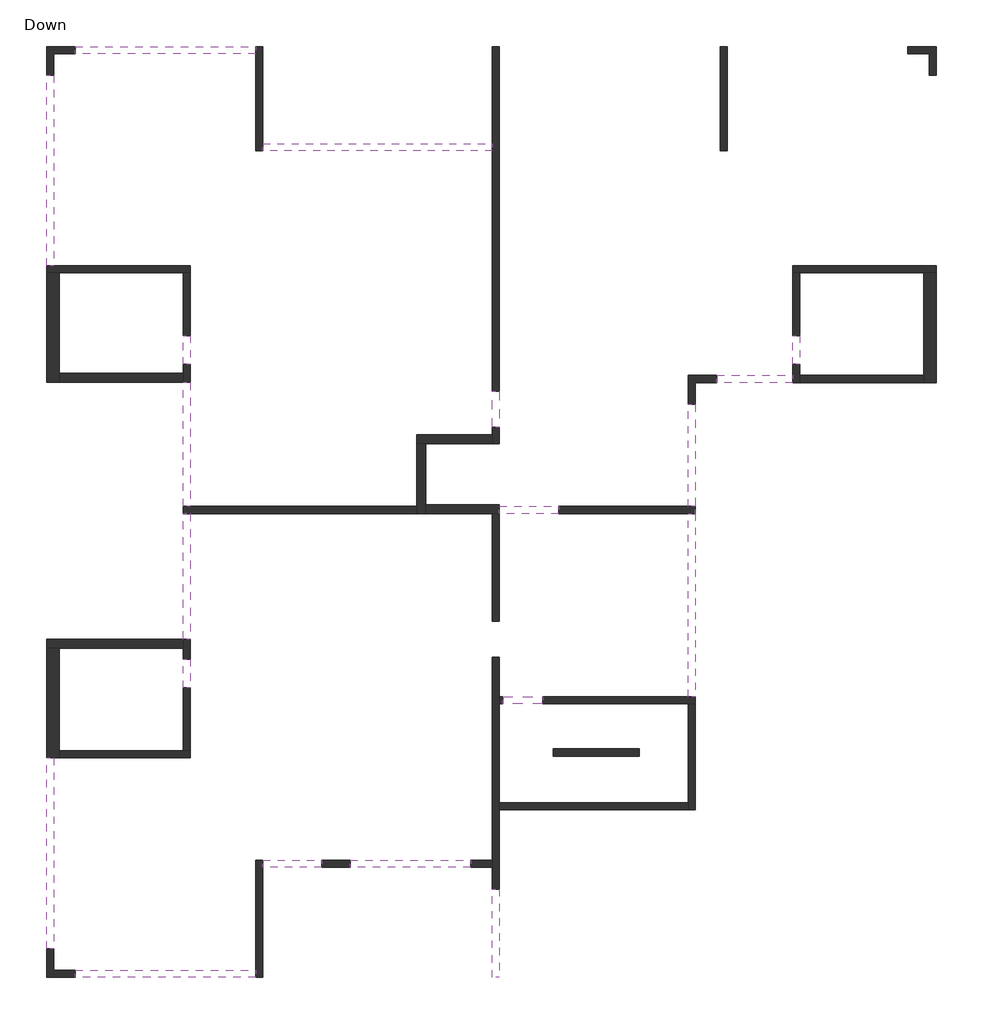
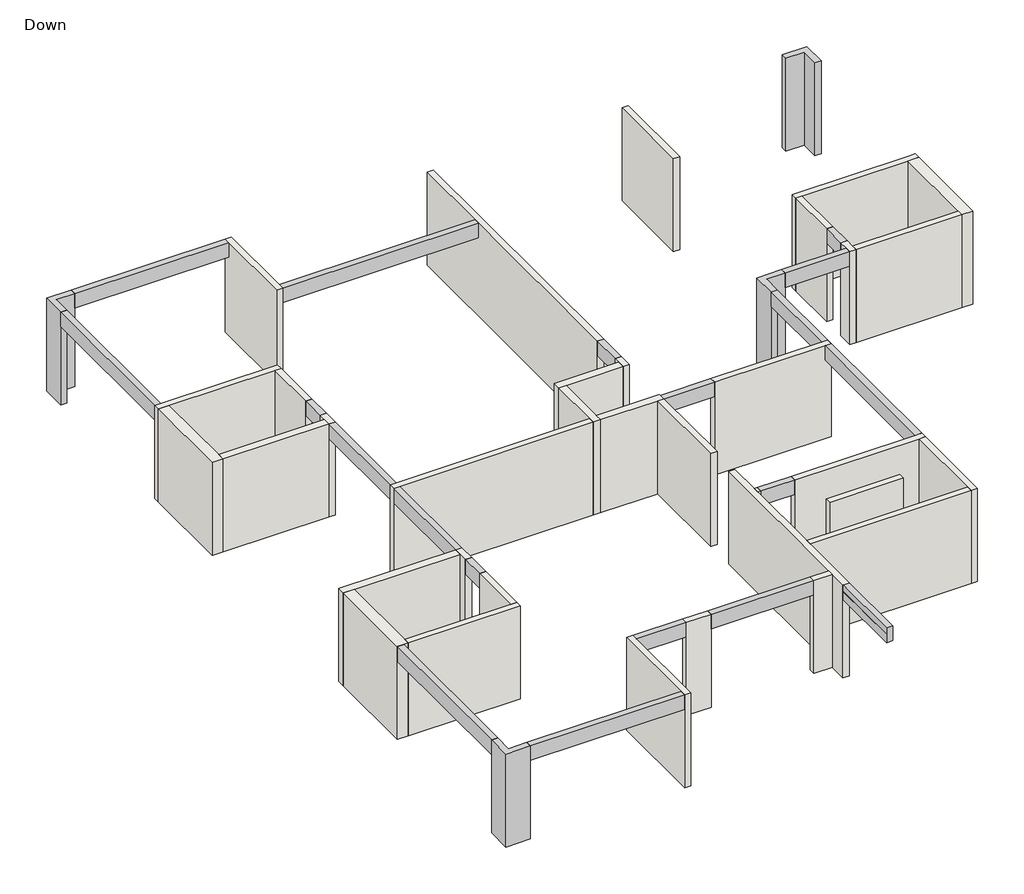
# One storey: 34 walls, 19 beams, 4 columns.
# Revit data of these elements (continued)
# Element 30 (IfcWall, "20") (continued)
#   Base Constraint = Down
#   Top Constraint = Typical Floor
#   Materials on its faces: "Concrete"
# Element 31 (IfcWall, "20")
#   Comments = ""
#   Mark = "W8"
#   SOFiSTiK_EdgeZones = "W8"
#   SOFiSTiK_AMG_Comments = ""
#   Top Offset = 0 cm
#   Base Offset = 0 cm
#   wall height = 320 cm
#   SOFiSTiK_AMG_Scheduled = yes
#   SOFiSTiK_AMG_Adjusted = yes
#   Phase Created = New Construction
#   Base Constraint = Down
#   Top Constraint = Typical Floor
#   Materials on its faces: "Concrete"
# Element 32 (IfcWall, "20")
#   Comments = ""
#   Mark = "W9"
#   SOFiSTiK_EdgeZones = "W9"
#   SOFiSTiK_AMG_Comments = ""
#   Top Offset = 0 cm
#   Base Offset = 0 cm
#   wall height = 320 cm
#   SOFiSTiK_AMG_Scheduled = yes
#   SOFiSTiK_AMG_Adjusted = yes
#   Phase Created = New Construction
#   Base Constraint = Down
#   Top Constraint = Typical Floor
#   Materials on its faces: "Concrete"
# Element 33 (IfcWall, "20")
#   Comments = ""
#   Mark = "W10"
#   SOFiSTiK_EdgeZones = "W10"
#   SOFiSTiK_AMG_Comments = ""
#   Top Offset = 0 cm
#   Base Offset = 0 cm
#   wall height = 320 cm
#   SOFiSTiK_AMG_Scheduled = yes
#   SOFiSTiK_AMG_Adjusted = yes
#   Phase Created = New Construction
#   Base Constraint = Down
#   Top Constraint = Typical Floor
#   Materials on its faces: "Concrete"
# Element 34 (IfcWall, "20")
#   Comments = ""
#   Mark = "W11"
#   SOFiSTiK_EdgeZones = "W11"
#   SOFiSTiK_AMG_Comments = ""
#   Top Offset = 0 cm
#   Base Offset = 0 cm
#   wall height = 320 cm
#   SOFiSTiK_AMG_Scheduled = yes
#   SOFiSTiK_AMG_Adjusted = yes
#   Phase Created = New Construction
#   Base Constraint = Down
#   Top Constraint = Typical Floor
#   Materials on its faces: "Concrete"
# Element 35 (IfcWall, "20")
#   Comments = ""
#   Mark = "W12"
#   SOFiSTiK_EdgeZones = "W12"
#   SOFiSTiK_AMG_Comments = ""
#   Top Offset = 0 cm
#   Base Offset = 0 cm
#   wall height = 320 cm
#   SOFiSTiK_AMG_Scheduled = yes
#   SOFiSTiK_AMG_Adjusted = yes
#   Phase Created = New Construction
#   Base Constraint = Down
#   Top Constraint = Typical Floor
#   Materials on its faces: "Concrete"
# Element 36 (IfcWall, "20")
#   Comments = ""
#   Mark = "W13"
#   SOFiSTiK_EdgeZones = "W13"
#   SOFiSTiK_AMG_Comments = ""
#   Top Offset = 0 cm
#   Base Offset = 0 cm
#   wall height = 320 cm
#   SOFiSTiK_AMG_Scheduled = yes
#   SOFiSTiK_AMG_Adjusted = yes
#   Phase Created = New Construction
#   Base Constraint = Down
#   Top Constraint = Typical Floor
#   Materials on its faces: "Concrete"
# Element 37 (IfcWall, "20")
#   Comments = ""
#   Mark = "W14"
#   SOFiSTiK_EdgeZones = "W14"
#   SOFiSTiK_AMG_Comments = ""
#   Top Offset = 0 cm
#   Base Offset = 0 cm
#   wall height = 320 cm
#   SOFiSTiK_AMG_Scheduled = yes
#   SOFiSTiK_AMG_Adjusted = yes
#   Phase Created = New Construction
#   Base Constraint = Down
#   Top Constraint = Typical Floor
#   Materials on its faces: "Concrete"
# Element 38 (IfcWall, "20")
#   Comments = ""
#   Mark = "W15"
#   SOFiSTiK_EdgeZones = "W15"
#   SOFiSTiK_AMG_Comments = ""
#   Top Offset = 0 cm
#   Base Offset = 0 cm
#   wall height = 320 cm
#   SOFiSTiK_AMG_Scheduled = yes
#   SOFiSTiK_AMG_Adjusted = yes
#   Phase Created = New Construction
#   Base Constraint = Down
#   Top Constraint = Typical Floor
#   Materials on its faces: "Concrete"
# Element 39 (IfcWall, "20")
#   Comments = ""
#   Mark = "W16"
#   SOFiSTiK_EdgeZones = "W16"
#   SOFiSTiK_AMG_Comments = ""
#   Top Offset = 0 cm
#   Base Offset = 0 cm
#   wall height = 320 cm
#   SOFiSTiK_AMG_Scheduled = yes
#   SOFiSTiK_AMG_Adjusted = yes
#   Phase Created = New Construction
#   Base Constraint = Down
#   Top Constraint = Typical Floor
#   Materials on its faces: "Concrete"
# Element 40 (IfcWall, "20")
#   Comments = ""
#   Mark = "W17"
#   SOFiSTiK_EdgeZones = "W17"
#   SOFiSTiK_AMG_Comments = ""
#   Top Offset = 0 cm
#   Base Offset = 0 cm
#   wall height = 320 cm
#   SOFiSTiK_AMG_Scheduled = yes
#   SOFiSTiK_AMG_Adjusted = yes
#   Phase Created = New Construction
#   Base Constraint = Down
#   Top Constraint = Typical Floor
#   Materials on its faces: "Concrete"
# Element 41 (IfcWall, "20")
#   Comments = ""
#   Mark = "W18"
#   SOFiSTiK_EdgeZones = "W18"
#   SOFiSTiK_AMG_Comments = ""
#   Top Offset = 0 cm
#   Base Offset = 0 cm
#   wall height = 320 cm
#   SOFiSTiK_AMG_Scheduled = yes
#   SOFiSTiK_AMG_Adjusted = yes
#   Phase Created = New Construction
#   Base Constraint = Down
#   Top Constraint = Typical Floor
#   Materials on its faces: "Concrete"
# Element 42 (IfcWall, "20")
#   Comments = ""
#   Mark = "W19"
#   SOFiSTiK_EdgeZones = "W19"
#   SOFiSTiK_AMG_Comments = "Too Short /"
#   Top Offset = 0 cm
#   Base Offset = 0 cm
#   wall height = 320 cm
#   SOFiSTiK_AMG_Scheduled = yes
#   SOFiSTiK_AMG_Adjusted = yes
#   Phase Created = New Construction
#   Base Constraint = Down
#   Top Constraint = Typical Floor
#   Materials on its faces: "Concrete"
# Element 43 (IfcWall, "20")
#   Comments = ""
#   Mark = "W20"
#   SOFiSTiK_EdgeZones = "W20"
#   SOFiSTiK_AMG_Comments = ""
#   Top Offset = 0 cm
#   Base Offset = 0 cm
#   wall height = 320 cm
#   SOFiSTiK_AMG_Scheduled = yes
#   SOFiSTiK_AMG_Adjusted = yes
#   Phase Created = New Construction
#   Base Constraint = Down
#   Top Constraint = Typical Floor
#   Materials on its faces: "Concrete"
# Element 44 (IfcWall, "20")
#   Comments = ""
#   Mark = "W21"
#   SOFiSTiK_EdgeZones = "W21"
#   SOFiSTiK_AMG_Comments = ""
#   Top Offset = 0 cm
#   Base Offset = 0 cm
#   wall height = 320 cm
#   SOFiSTiK_AMG_Scheduled = yes
#   SOFiSTiK_AMG_Adjusted = yes
#   Phase Created = New Construction
#   Base Constraint = Down
#   Top Constraint = Typical Floor
#   Materials on its faces: "Concrete"
# Element 45 (IfcWall, "20")
#   Comments = ""
#   Mark = "W22"
#   SOFiSTiK_EdgeZones = "W22"
#   SOFiSTiK_AMG_Comments = ""
#   Top Offset = 0 cm
#   Base Offset = 0 cm
#   wall height = 320 cm
#   SOFiSTiK_AMG_Scheduled = yes
#   SOFiSTiK_AMG_Adjusted = yes
#   Phase Created = New Construction
#   Base Constraint = Down
#   Top Constraint = Typical Floor
#   Materials on its faces: "Concrete"
# Element 46 (IfcWall, "20")
#   Comments = ""
#   Mark = "W23"
#   SOFiSTiK_EdgeZones = "W23"
#   SOFiSTiK_AMG_Comments = ""
#   Top Offset = 0 cm
#   Base Offset = 0 cm
#   wall height = 320 cm
#   SOFiSTiK_AMG_Scheduled = yes
#   SOFiSTiK_AMG_Adjusted = yes
#   Phase Created = New Construction
#   Base Constraint = Down
#   Top Constraint = Typical Floor
#   Materials on its faces: "Concrete"
# Element 47 (IfcWall, "20")
#   Comments = ""
#   Mark = "W24"
#   SOFiSTiK_EdgeZones = "W24"
#   SOFiSTiK_AMG_Comments = ""
#   Top Offset = 0 cm
#   Base Offset = 0 cm
#   wall height = 320 cm
#   SOFiSTiK_AMG_Scheduled = yes
#   SOFiSTiK_AMG_Adjusted = yes
#   Phase Created = New Construction
#   Base Constraint = Down
#   Top Constraint = Typical Floor
#   Materials on its faces: "Concrete"
# Element 48 (IfcWall, "20")
#   Comments = ""
#   Mark = "W25"
#   SOFiSTiK_EdgeZones = "W25"
#   SOFiSTiK_AMG_Comments = ""
#   Top Offset = 0 cm
#   Base Offset = 0 cm
#   wall height = 320 cm
#   SOFiSTiK_AMG_Scheduled = yes
#   SOFiSTiK_AMG_Adjusted = yes
#   Phase Created = New Construction
#   Base Constraint = Down
#   Top Constraint = Typical Floor
#   Materials on its faces: "Concrete"
# Element 49 (IfcWall, "20")
#   Comments = ""
#   Mark = "W26"
#   SOFiSTiK_EdgeZones = "W26"
#   SOFiSTiK_AMG_Comments = ""
#   Top Offset = 0 cm
#   Base Offset = 0 cm
#   wall height = 320 cm
#   SOFiSTiK_AMG_Scheduled = yes
#   SOFiSTiK_AMG_Adjusted = yes
#   Phase Created = New Construction
#   Base Constraint = Down
#   Top Constraint = Typical Floor
#   Materials on its faces: "Concrete"
# Element 50 (IfcWall, "25")
#   Comments = ""
#   Mark = "W30"
#   SOFiSTiK_EdgeZones = "W30"
#   SOFiSTiK_AMG_Comments = ""
#   Top Offset = 0 cm
#   Base Offset = 0 cm
#   wall height = 320 cm
#   SOFiSTiK_AMG_Scheduled = yes
#   SOFiSTiK_AMG_Adjusted = yes
#   Phase Created = New Construction
#   Base Constraint = Down
#   Top Constraint = Typical Floor
#   Materials on its faces: "Concrete"
# Element 51 (IfcWall, "25")
#   Comments = ""
#   Mark = "W31"
#   SOFiSTiK_EdgeZones = "W31"
#   SOFiSTiK_AMG_Comments = ""
#   Top Offset = 0 cm
#   Base Offset = 0 cm
#   wall height = 320 cm
#   SOFiSTiK_AMG_Scheduled = yes
#   SOFiSTiK_AMG_Adjusted = yes
#   Phase Created = New Construction
#   Base Constraint = Down
#   Top Constraint = Typical Floor
#   Materials on its faces: "Concrete"
# Element 52 (IfcWall, "25")
#   Comments = ""
#   Mark = "W32"
#   SOFiSTiK_EdgeZones = "W32"
#   SOFiSTiK_AMG_Comments = ""
#   Top Offset = 0 cm
#   Base Offset = 0 cm
#   wall height = 320 cm
#   SOFiSTiK_AMG_Scheduled = yes
#   SOFiSTiK_AMG_Adjusted = yes
#   Phase Created = New Construction
#   Base Constraint = Down
#   Top Constraint = Typical Floor
#   Materials on its faces: "Concrete"
# Element 53 (IfcWall, "25")
#   Comments = ""
#   Mark = "W33"
#   SOFiSTiK_EdgeZones = "W33"
#   SOFiSTiK_AMG_Comments = ""
#   Top Offset = 0 cm
#   Base Offset = 0 cm
#   wall height = 320 cm
#   SOFiSTiK_AMG_Scheduled = yes
#   SOFiSTiK_AMG_Adjusted = yes
#   Phase Created = New Construction
#   Base Constraint = Down
#   Top Constraint = Typical Floor
#   Materials on its faces: "Concrete"
# Element 54 (IfcWall, "25")
#   Comments = ""
#   Mark = "W34"
#   SOFiSTiK_EdgeZones = "W34"
#   SOFiSTiK_AMG_Comments = ""
#   Top Offset = 0 cm
#   Base Offset = 0 cm
#   wall height = 320 cm
#   SOFiSTiK_AMG_Scheduled = yes
#   SOFiSTiK_AMG_Adjusted = yes
#   Phase Created = New Construction
#   Base Constraint = Down
#   Top Constraint = Typical Floor
#   Materials on its faces: "Concrete"
# Element 55 (IfcWall, "35")
#   Comments = ""
#   Mark = "W27"
#   SOFiSTiK_EdgeZones = "W27"
#   SOFiSTiK_AMG_Comments = ""
#   Top Offset = 0 cm
#   Base Offset = 0 cm
#   wall height = 320 cm
#   SOFiSTiK_AMG_Scheduled = yes
#   SOFiSTiK_AMG_Adjusted = yes
#   Phase Created = New Construction
#   Base Constraint = Down
#   Top Constraint = Typical Floor
#   Materials on its faces: "Concrete"
# Element 56 (IfcWall, "35")
#   Comments = ""
#   Mark = "W28"
#   SOFiSTiK_EdgeZones = "W28"
#   SOFiSTiK_AMG_Comments = ""
#   Top Offset = 0 cm
#   Base Offset = 0 cm
#   wall height = 320 cm
#   SOFiSTiK_AMG_Scheduled = yes
#   SOFiSTiK_AMG_Adjusted = yes
#   Phase Created = New Construction
#   Base Constraint = Down
#   Top Constraint = Typical Floor
#   Materials on its faces: "Concrete"
# Element 57 (IfcWall, "35")
#   Comments = ""
#   Mark = "W29"
#   SOFiSTiK_EdgeZones = "W29"
#   SOFiSTiK_AMG_Comments = ""
#   Top Offset = 0 cm
#   Base Offset = 0 cm
#   wall height = 320 cm
#   SOFiSTiK_AMG_Scheduled = yes
#   SOFiSTiK_AMG_Adjusted = yes
#   Phase Created = New Construction
#   Base Constraint = Down
#   Top Constraint = Typical Floor
#   Materials on its faces: "Concrete"
# Materials
#   "Concrete": class "Concrete", colour RGB 192 192 192, transparency 0, Keynote = "01000", Description = "Cast-in-place concrete", Cost = 0
#   "Concrete, Cast-in-Place gray": class "Concrete", colour RGB 192 192 192, transparency 0, Description = "Cast-in-place concrete", Cost = 0
